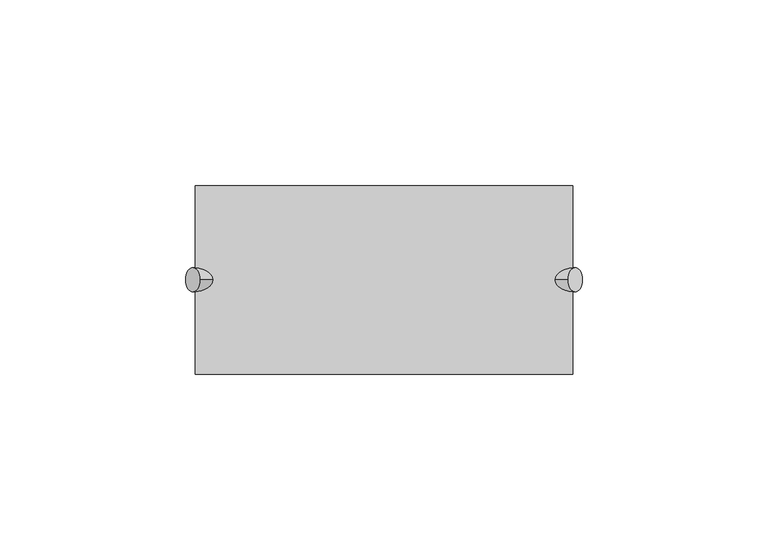
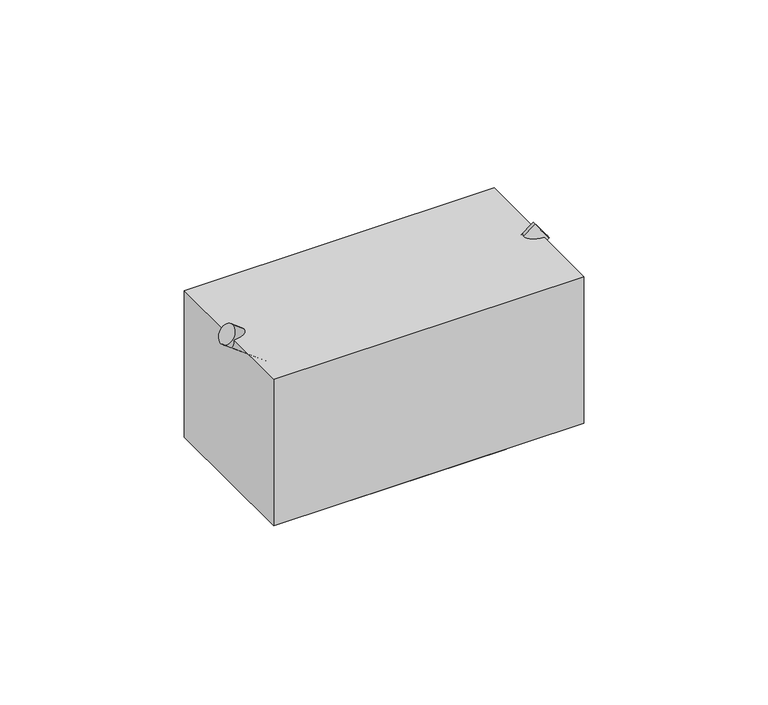
"""IFC4 building model written with IfcOpenShell, lengths in millimetres: proxy geometry, A5145 - Hook, Garment, Double : A5145 - Hook, Garment, Double."""

import ifcopenshell
import ifcopenshell.guid

model = None  # the IFC model being written
_history = None  # IfcOwnerHistory: only IFC2X3 demands one
_inside = {}  # id of a spatial element -> (the spatial element, [elements in it])
_under = {}  # id of a project, library or spatial element -> (it, [spatial elements below it])
_declared = {}  # id of a project -> (the project, [libraries it declares])
_typed = {}  # id of a type object -> (the type object, [elements of that type])
_made_of = {}  # id of a material, layer set ... -> (it, [elements and type objects made of it])


def new_model(schema):
    """Start an empty IFC model of exactly this schema.

    Asked for "IFC4X3", IfcOpenShell would pick the latest addendum, in which some entities
    have other attributes; the version numbers below select the first issue.
    IFC2X3 requires an IfcOwnerHistory on every rooted entity: one is made here for all.
    """
    global model, _history
    if schema == "IFC4X3":
        model = ifcopenshell.file(schema_version=(4, 3, 0, 0))
    else:
        model = ifcopenshell.file(schema=schema)
    _inside.clear()
    _under.clear()
    _declared.clear()
    _typed.clear()
    _made_of.clear()
    _history = None
    if model.schema == "IFC2X3":
        org = make("IfcOrganization", Name="unknown")
        user = make(
            "IfcPersonAndOrganization",
            ThePerson=make("IfcPerson", FamilyName="unknown"),
            TheOrganization=org,
        )
        app = make(
            "IfcApplication",
            ApplicationDeveloper=org,
            Version="unknown",
            ApplicationFullName="unknown",
            ApplicationIdentifier="unknown",
        )
        _history = make(
            "IfcOwnerHistory",
            OwningUser=user,
            OwningApplication=app,
            ChangeAction="ADDED",
            CreationDate=0,
        )
    return model


def make(cls, **values):
    """One entity of the class cls with the attributes given. An attribute that is None is left unset."""
    return model.create_entity(
        cls, **{name: value for name, value in values.items() if value is not None}
    )


def rooted(cls, **values):
    """An entity with a GlobalId (a new one), such as an element, a storey or a relation."""
    return make(cls, GlobalId=ifcopenshell.guid.new(), OwnerHistory=_history, **values)


def si_unit(unit_type, name, prefix=None):
    """IfcSIUnit, for example si_unit("LENGTHUNIT", "METRE", prefix="MILLI")."""
    return make("IfcSIUnit", UnitType=unit_type, Prefix=prefix, Name=name)


def assignment(units):
    """IfcUnitAssignment: the units of a project."""
    return None if units is None else make("IfcUnitAssignment", Units=units)


def point(xyz):
    """IfcCartesianPoint."""
    return None if xyz is None else make("IfcCartesianPoint", Coordinates=xyz)


def direction(xyz):
    """IfcDirection."""
    return None if xyz is None else make("IfcDirection", DirectionRatios=xyz)


def frame(location, z_axis=None, x_axis=None):
    """IfcAxis2Placement3D, a coordinate frame: its origin and axes. An axis left out is left unset."""
    return make(
        "IfcAxis2Placement3D",
        Location=point(location),
        Axis=direction(z_axis),
        RefDirection=direction(x_axis),
    )


def origin():
    """The frame at (0, 0, 0) with its axes left unset."""
    return frame((0.0, 0.0, 0.0))


def origin_with_axes():
    """The frame at (0, 0, 0) with the z axis (0, 0, 1) and the x axis (1, 0, 0) written out."""
    return frame((0.0, 0.0, 0.0), z_axis=(0.0, 0.0, 1.0), x_axis=(1.0, 0.0, 0.0))


def place(relative_to, where):
    """IfcLocalPlacement: puts the frame where relative to a parent placement (None: the world)."""
    return make(
        "IfcLocalPlacement", PlacementRelTo=relative_to, RelativePlacement=where
    )


def context(
    kind, dimensions, precision=None, world=None, true_north=None, identifier=None
):
    """IfcGeometricRepresentationContext, for example the 3D "Model" context."""
    return make(
        "IfcGeometricRepresentationContext",
        ContextIdentifier=identifier,
        ContextType=kind,
        CoordinateSpaceDimension=dimensions,
        Precision=precision,
        WorldCoordinateSystem=world,
        TrueNorth=true_north,
    )


def project(units=None, contexts=None):
    """IfcProject with its units and contexts."""
    return rooted(
        "IfcProject",
        Name="project",
        RepresentationContexts=contexts,
        UnitsInContext=assignment(units),
    )


def spatial(cls, under=None, at=None, **own):
    """A site, building, storey or space (cls), placed at a placement, below another one or the project."""
    s = rooted(cls, ObjectPlacement=at, **own)
    if under is not None:
        _under.setdefault(under.id(), (under, []))[1].append(s)
    return s


def polyline(points):
    """IfcPolyline through the points."""
    return make("IfcPolyline", Points=[point(p) for p in points])


def circle_curve(where, radius):
    """IfcCircle in the frame where."""
    return make("IfcCircle", Position=where, Radius=radius)


def ellipse_curve(where, semi_axis1, semi_axis2):
    """IfcEllipse in the frame where."""
    return make(
        "IfcEllipse", Position=where, SemiAxis1=semi_axis1, SemiAxis2=semi_axis2
    )


def outline(outer, holes=None, kind="AREA"):
    """IfcArbitraryClosedProfileDef: a profile drawn as a closed curve; with holes, ...WithVoids."""
    if holes is None:
        return make("IfcArbitraryClosedProfileDef", ProfileType=kind, OuterCurve=outer)
    return make(
        "IfcArbitraryProfileDefWithVoids",
        ProfileType=kind,
        OuterCurve=outer,
        InnerCurves=holes,
    )


def extrude(swept, where, along, depth):
    """IfcExtrudedAreaSolid: the profile swept, set in the frame where, extruded along a direction by depth."""
    return make(
        "IfcExtrudedAreaSolid",
        SweptArea=swept,
        Position=where,
        ExtrudedDirection=direction(along),
        Depth=depth,
    )


def shape(context_of_items, identifier, shape_type, items):
    """IfcShapeRepresentation: the items that make up one representation, for example the "Body"."""
    return make(
        "IfcShapeRepresentation",
        ContextOfItems=context_of_items,
        RepresentationIdentifier=identifier,
        RepresentationType=shape_type,
        Items=items,
    )


def source(mapping_origin, context_of_items, identifier, shape_type, items):
    """IfcRepresentationMap: a shape defined once, which mapped items show again and again."""
    return make(
        "IfcRepresentationMap",
        MappingOrigin=mapping_origin,
        MappedRepresentation=shape(context_of_items, identifier, shape_type, items),
    )


def transform(
    local_origin,
    x_axis=None,
    y_axis=None,
    z_axis=None,
    scale=None,
    scale2=None,
    scale3=None,
    uniform=True,
):
    """IfcCartesianTransformationOperator3D, or its non-uniform kind. x_axis, y_axis, z_axis: its Axis1, 2, 3."""
    if uniform:
        return make(
            "IfcCartesianTransformationOperator3D",
            Axis1=direction(x_axis),
            Axis2=direction(y_axis),
            LocalOrigin=point(local_origin),
            Scale=scale,
            Axis3=direction(z_axis),
        )
    return make(
        "IfcCartesianTransformationOperator3DnonUniform",
        Axis1=direction(x_axis),
        Axis2=direction(y_axis),
        LocalOrigin=point(local_origin),
        Scale=scale,
        Axis3=direction(z_axis),
        Scale2=scale2,
        Scale3=scale3,
    )


def mapped(mapping_source, mapping_target):
    """IfcMappedItem: shows the shape of a source again, moved by a transform."""
    return make(
        "IfcMappedItem", MappingSource=mapping_source, MappingTarget=mapping_target
    )


def made_of(thing, what):
    """Note that an element or type object is made of a material, layer set ...; save() writes the relation."""
    if what is not None:
        _made_of.setdefault(what.id(), (what, []))[1].append(thing)
    return thing


def element(
    cls,
    number,
    at=None,
    inside=None,
    cuts=None,
    type_object=None,
    material=None,
    context=None,
    identifier="Body",
    shape_type=None,
    held_by="IfcProductDefinitionShape",
    body=None,
    shapes=None,
    **own,
):
    """One element of the class cls, such as IfcWall. Its Tag is "e" and its number.

    at: its placement. inside: the storey or other place that contains it. cuts: it is an
    opening in that element (IfcRelVoidsElement). A single representation is given by context,
    identifier, shape_type and body (its items); several are given by shapes. held_by: the class
    of the entity that holds the representations. save() writes the other relations.
    """
    e = rooted(cls, Tag="e%d" % number, ObjectPlacement=at, **own)
    if body is not None:
        shapes = [shape(context, identifier, shape_type, body)]
    if shapes is not None:
        e.Representation = make(held_by, Representations=shapes)
    if inside is not None:
        _inside.setdefault(inside.id(), (inside, []))[1].append(e)
    if cuts is not None:
        rooted(
            "IfcRelVoidsElement", RelatingBuildingElement=cuts, RelatedOpeningElement=e
        )
    if type_object is not None:
        _typed.setdefault(type_object.id(), (type_object, []))[1].append(e)
    return made_of(e, material)


def aggregate(whole, parts):
    """IfcRelAggregates: a whole, such as a stair, and the parts it consists of."""
    return rooted("IfcRelAggregates", RelatingObject=whole, RelatedObjects=parts)


def save(model, path):
    """Write the relations noted so far, then the file.

    IfcRelAggregates (storeys below a building ...), IfcRelContainedInSpatialStructure (elements
    in a storey), IfcRelDefinesByType, IfcRelAssociatesMaterial and IfcRelDeclares: one each for
    every whole, place, type object, material and project.
    """
    for whole, parts in _under.values():
        aggregate(whole, parts)
    for where, things in _inside.values():
        rooted(
            "IfcRelContainedInSpatialStructure",
            RelatedElements=things,
            RelatingStructure=where,
        )
    for kind, things in _typed.values():
        rooted("IfcRelDefinesByType", RelatedObjects=things, RelatingType=kind)
    for what, things in _made_of.values():
        rooted("IfcRelAssociatesMaterial", RelatedObjects=things, RelatingMaterial=what)
    for by, libraries in _declared.values():
        rooted("IfcRelDeclares", RelatingContext=by, RelatedDefinitions=libraries)
    model.write(path)


def plane_surface(at):
    """IfcPlane: the flat surface through the origin of the frame at, square to its z axis."""
    return make("IfcPlane", Position=at)


def cylinder_surface(at, radius):
    """IfcCylindricalSurface: all points at the distance radius from the z axis of the frame at."""
    return make("IfcCylindricalSurface", Position=at, Radius=radius)


def advanced_brep(points, edges, surfaces, faces):
    """IfcAdvancedBrep: a solid bounded by faces that lie on surfaces and meet in shared edges.

    An edge is (start, end): straight between two places in points (the first is 0);
    or (start, end, curve); or (start, end, curve, False) where it runs against its curve.
    A face is (place in surfaces, loops), or (place, loops, False) where it looks against
    its surface's normal. A loop lists edges by number (the first is 1), with a minus sign
    where the edge is run from its end to its start. The first loop is the outer one.
    """
    corners = [point(p) for p in points]
    vertices = [make("IfcVertexPoint", VertexGeometry=c) for c in corners]
    made = []
    for start, end, *more in edges:
        made.append(
            make(
                "IfcEdgeCurve",
                EdgeStart=vertices[start],
                EdgeEnd=vertices[end],
                EdgeGeometry=more[0] if more else make("IfcPolyline", Points=[corners[start], corners[end]]),
                SameSense=more[1] if len(more) > 1 else True,
            )
        )
    hull = []
    for where, loops, *sense in faces:
        bounds = []
        for j, loop in enumerate(loops):
            ring = [make("IfcOrientedEdge", EdgeElement=made[abs(k) - 1], Orientation=k > 0) for k in loop]
            bounds.append(
                make(
                    "IfcFaceOuterBound" if j == 0 else "IfcFaceBound",
                    Bound=make("IfcEdgeLoop", EdgeList=ring),
                    Orientation=True,
                )
            )
        hull.append(make("IfcAdvancedFace", Bounds=bounds, FaceSurface=surfaces[where], SameSense=sense[0] if sense else True))
    return make("IfcAdvancedBrep", Outer=make("IfcClosedShell", CfsFaces=hull))


def specialty_equipment_4be3cf79(model_context):
    return source(origin(), model_context, "Body", "SolidModel", [
        extrude(outline(polyline([(50.8, 25.4), (50.8, -25.4), (-50.8, -25.4), (-50.8, 25.4), (50.8, 25.4)])), origin_with_axes(), (0.0, 0.0, 1.0), 50.8),
        advanced_brep(
        [(-53.475253, 0.0, 48.7696452), (-49.5999303, 0.0, 53.9367422), (-5.3823927, 0.0, 12.7), (0.0, -3.2294356, 12.7), (0.0, 0.0, 16.7367945), (0.0, 3.2294356, 12.7), (53.475253, 0.0, 48.7696452), (49.5999303, 0.0, 53.9367422), (5.3823927, 0.0, 12.7), (-25.4, -25.4, 12.7), (25.4, -25.4, 12.7), (25.4, 25.4, 12.7), (-25.4, 25.4, 12.7), (-25.4, -25.4, 0.0), (-25.4, 25.4, 0.0), (25.4, 25.4, 0.0), (25.4, -25.4, 0.0)],
        [
            (0, 1, circle_curve(frame((-51.5375917, 0.0, 51.3531937), z_axis=(-0.7999999999999928, 0.0, 0.6000000000000097), x_axis=(0.6000000000000097, 0.0, 0.7999999999999928)), 3.2294356)),
            (1, 0, circle_curve(frame((-51.5375917, 0.0, 51.3531937), z_axis=(-0.7999999999999928, 0.0, 0.6000000000000097), x_axis=(0.6000000000000097, 0.0, 0.7999999999999928)), 3.2294356)),
            (0, 2),
            (2, 3, ellipse_curve(frame((0.0, 0.0, 12.7), z_axis=(0.0, 0.0, 1.0), x_axis=(-0.9999999999999999, 0.0, 0.0)), 5.3823927, 3.2294356)),
            (3, 4, ellipse_curve(frame((0.0, 0.0, 12.7), z_axis=(-0.9999999999999999, 0.0, 0.0), x_axis=(0.0, 0.0, 1.0)), 4.0367945, 3.2294356)),
            (4, 1),
            (4, 5, ellipse_curve(frame((0.0, 0.0, 12.7), z_axis=(-0.9999999999999999, 0.0, 0.0), x_axis=(0.0, 0.0, 1.0)), 4.0367945, 3.2294356)),
            (5, 2, ellipse_curve(frame((0.0, 0.0, 12.7), z_axis=(0.0, 0.0, 1.0), x_axis=(-0.9999999999999999, 0.0, 0.0)), 5.3823927, 3.2294356)),
            (6, 7, circle_curve(frame((51.5375917, 0.0, 51.3531937), z_axis=(0.7999999999999928, 0.0, 0.6000000000000097), x_axis=(-0.6000000000000097, 0.0, 0.7999999999999928)), 3.2294356)),
            (7, 6, circle_curve(frame((51.5375917, 0.0, 51.3531937), z_axis=(0.7999999999999928, 0.0, 0.6000000000000097), x_axis=(-0.6000000000000097, 0.0, 0.7999999999999928)), 3.2294356)),
            (7, 4),
            (3, 8, ellipse_curve(frame((0.0, 0.0, 12.7), z_axis=(0.0, 0.0, 1.0), x_axis=(0.9999999999999999, 0.0, 0.0)), 5.3823927, 3.2294356)),
            (8, 6),
            (8, 5, ellipse_curve(frame((0.0, 0.0, 12.7), z_axis=(0.0, 0.0, 1.0), x_axis=(0.9999999999999999, 0.0, 0.0)), 5.3823927, 3.2294356)),
            (9, 10),
            (10, 11),
            (11, 12),
            (12, 9),
            (13, 14),
            (14, 15),
            (15, 16),
            (16, 13),
            (12, 14),
            (13, 9),
            (11, 15),
            (10, 16),
        ],
        [
            plane_surface(frame((-49.5999303, 0.0, 53.9367422), z_axis=(-0.7999999999999927, 0.0, 0.6000000000000097), x_axis=(0.0, 1.0, 0.0))),
            cylinder_surface(frame((0.0, 0.0, 12.7), z_axis=(-0.7999999999999928, 0.0, 0.6000000000000097), x_axis=(0.6000000000000097, 0.0, 0.7999999999999928)), 3.2294356),
            plane_surface(frame((49.5999303, 0.0, 53.9367422), z_axis=(0.7999999999999927, 0.0, 0.6000000000000097), x_axis=(0.0, -1.0, 0.0))),
            cylinder_surface(frame((0.0, 0.0, 12.7), z_axis=(0.7999999999999928, 0.0, 0.6000000000000097), x_axis=(-0.6000000000000097, 0.0, 0.7999999999999928)), 3.2294356),
            plane_surface(frame((25.4, -25.4, 12.7), z_axis=(0.0, 0.0, 1.0), x_axis=(1.0, 0.0, 0.0))),
            plane_surface(frame((25.4, -25.4, 0.0), z_axis=(0.0, 0.0, -1.0), x_axis=(-1.0, 0.0, 0.0))),
            plane_surface(frame((-25.4, 25.4, 12.7), z_axis=(-1.0, 0.0, 0.0), x_axis=(0.0, 0.0, -1.0))),
            plane_surface(frame((25.4, 25.4, 12.7), z_axis=(0.0, 1.0, 0.0), x_axis=(0.0, 0.0, -1.0))),
            plane_surface(frame((25.4, -25.4, 12.7), z_axis=(1.0, 0.0, 0.0), x_axis=(0.0, 0.0, -1.0))),
            plane_surface(frame((-25.4, -25.4, 12.7), z_axis=(0.0, -1.0, 0.0), x_axis=(0.0, 0.0, -1.0))),
        ],
        [
            (0, [[1, 2]]),
            (1, [[-1, 3, 4, 5, 6]]),
            (1, [[-2, -6, 7, 8, -3]]),
            (2, [[9, 10]]),
            (3, [[-10, 11, -5, 12, 13]]),
            (3, [[-9, -13, 14, -7, -11]]),
            (4, [[15, 16, 17, 18], [-4, -8, -14, -12]]),
            (5, [[19, 20, 21, 22]]),
            (6, [[-18, 23, -19, 24]]),
            (7, [[-17, 25, -20, -23]]),
            (8, [[-16, 26, -21, -25]]),
            (9, [[-15, -24, -22, -26]]),
        ],
    ),
    ])


if __name__ == "__main__":
    model = new_model("IFC4")
    model_context = context("Model", 3, world=origin())
    ifc_project = project(units=[si_unit("LENGTHUNIT", "METRE", prefix="MILLI")], contexts=[model_context])
    site = spatial("IfcSite", under=ifc_project)
    building = spatial("IfcBuilding", under=site)
    placement = place(None, origin())
    specialty_equipment_shape = specialty_equipment_4be3cf79(model_context)
    element("IfcBuildingElementProxy", 1, Name="A5145 - Hook, Garment, Double : A5145 - Hook, Garment, Double", ObjectType="A5145 - Hook, Garment, Double : A5145 - Hook, Garment, Double", at=placement, inside=building, context=model_context, shape_type="MappedRepresentation", body=[
        mapped(specialty_equipment_shape, transform((0.0, 0.0, 0.0), x_axis=(1.0, 0.0, 0.0), y_axis=(0.0, 1.0, 0.0), z_axis=(0.0, 0.0, 1.0))),
    ])
    save(model, "model.ifc")

# Revit data of these elements
# Type "A5145 - Hook, Garment, Double : A5145 - Hook, Garment, Double"
#   Watts2 = "0"
#   Watts1 = "0"
#   Unit_Issue = "EA"
#   UTIL_6_Misc = "-"
#   UTIL_5_NonMedGas = "-"
#   UTIL_4_MiscGas = "-"
#   UTIL_3_MedGas = "-"
#   UTIL_2_Elec = "-"
#   UTIL_1_WaterDrain = "-"
#   Nomenclature = "Hook, Garment, Double, SS, Surface Mounted"
#   NSN = "5340007541678"
#   Location [instance default] = ""
#   JSN = "A5145"
#   Fund_Source_VA = "-"
#   Fund_Source_Navy = "-"
#   Fund_Source_Army = "-"
#   Fund_Source_AF = "-"
#   ELEC_Volts2 = "0"
#   ELEC_Volts1 = "0"
#   ELEC_Phase2 = "0"
#   ELEC_Phase1 = "0"
#   ELEC_HertzSwitch = "0"
#   ELEC_HertzDependent = "0"
#   ELEC_Hertz = "0"
#   ELEC_Amps2 = "0"
#   ELEC_Amps1 = "0"
#   DetailDescription = "A surface mounted, satin finish stainless steel, double garment hook. Equipped with a concealed mounting bracket that is secured to a concealed wall plate. For general purpose use throughout the facility to hang various items of apparel."
#   CAT_VA = "A"
#   CAT_Navy = "A"
#   CAT_IHS = "-"
#   CAT_Army = "A"
#   CAT_AF = "A"
#   BTUperhour = "0"
#   Weight_IP = 0
#   Default Elevation = 4' - 0"
#   DIM_Width_IP = 0' - 4"
#   DIM_Height_IP = 0' - 2"
#   DIM_Depth_IP = 0' - 2"
#   Assembly Code = ""
# Element 1 (IfcBuildingElementProxy, "A5145 - Hook, Garment, Double : A5145 - Hook, Garment, Double")
#   Materials on its faces: "EquipSpace"
# Materials
#   "EquipSpace": class "Unassigned", colour RGB 221 217 195, transparency 0.5
